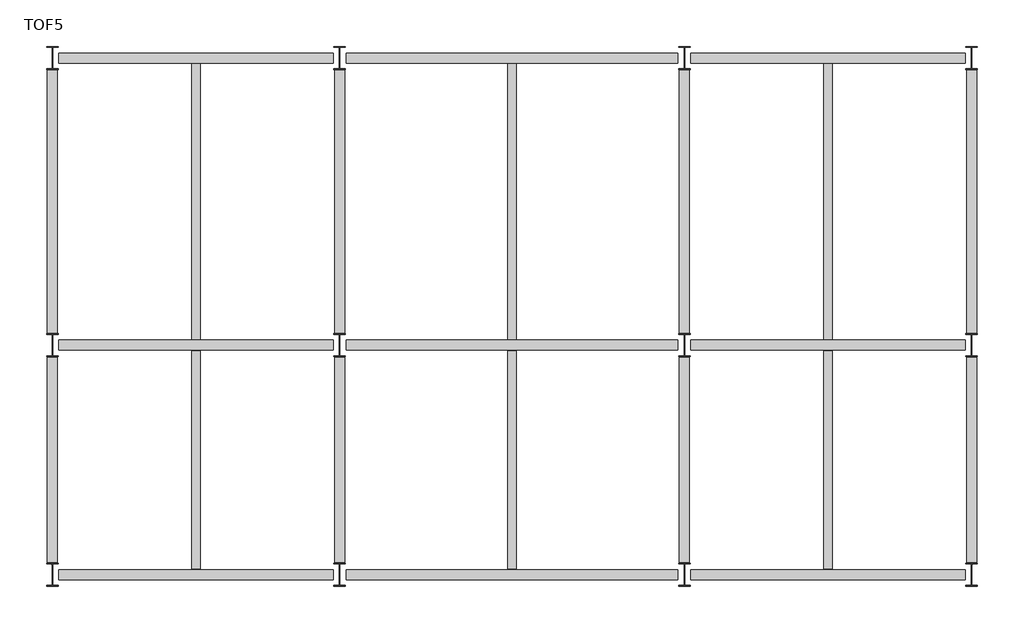
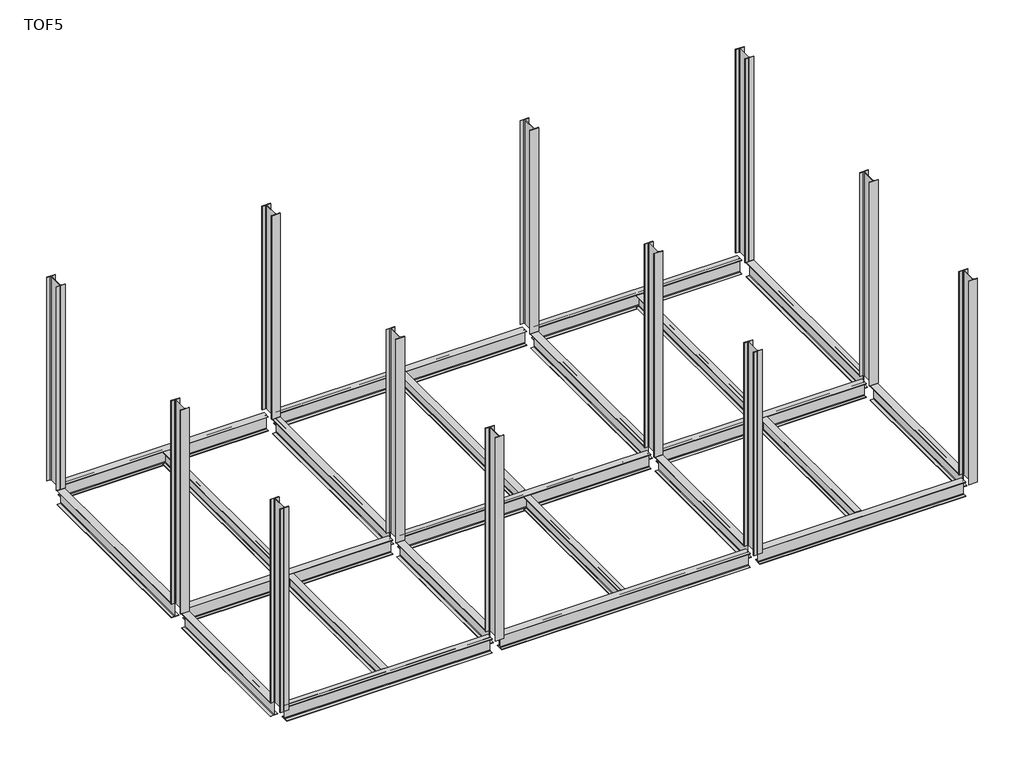
# One storey: 23 beams, 12 columns.
"""IFC4 building model written with IfcOpenShell, lengths in millimetres."""

import ifcopenshell
import ifcopenshell.guid

model = None  # the IFC model being written
_history = None  # IfcOwnerHistory: only IFC2X3 demands one
_inside = {}  # id of a spatial element -> (the spatial element, [elements in it])
_under = {}  # id of a project, library or spatial element -> (it, [spatial elements below it])
_declared = {}  # id of a project -> (the project, [libraries it declares])
_typed = {}  # id of a type object -> (the type object, [elements of that type])
_made_of = {}  # id of a material, layer set ... -> (it, [elements and type objects made of it])


def new_model(schema):
    """Start an empty IFC model of exactly this schema.

    Asked for "IFC4X3", IfcOpenShell would pick the latest addendum, in which some entities
    have other attributes; the version numbers below select the first issue.
    IFC2X3 requires an IfcOwnerHistory on every rooted entity: one is made here for all.
    """
    global model, _history
    if schema == "IFC4X3":
        model = ifcopenshell.file(schema_version=(4, 3, 0, 0))
    else:
        model = ifcopenshell.file(schema=schema)
    _inside.clear()
    _under.clear()
    _declared.clear()
    _typed.clear()
    _made_of.clear()
    _history = None
    if model.schema == "IFC2X3":
        org = make("IfcOrganization", Name="unknown")
        user = make(
            "IfcPersonAndOrganization",
            ThePerson=make("IfcPerson", FamilyName="unknown"),
            TheOrganization=org,
        )
        app = make(
            "IfcApplication",
            ApplicationDeveloper=org,
            Version="unknown",
            ApplicationFullName="unknown",
            ApplicationIdentifier="unknown",
        )
        _history = make(
            "IfcOwnerHistory",
            OwningUser=user,
            OwningApplication=app,
            ChangeAction="ADDED",
            CreationDate=0,
        )
    return model


def make(cls, **values):
    """One entity of the class cls with the attributes given. An attribute that is None is left unset."""
    return model.create_entity(
        cls, **{name: value for name, value in values.items() if value is not None}
    )


def rooted(cls, **values):
    """An entity with a GlobalId (a new one), such as an element, a storey or a relation."""
    return make(cls, GlobalId=ifcopenshell.guid.new(), OwnerHistory=_history, **values)


def si_unit(unit_type, name, prefix=None):
    """IfcSIUnit, for example si_unit("LENGTHUNIT", "METRE", prefix="MILLI")."""
    return make("IfcSIUnit", UnitType=unit_type, Prefix=prefix, Name=name)


def assignment(units):
    """IfcUnitAssignment: the units of a project."""
    return None if units is None else make("IfcUnitAssignment", Units=units)


def point(xyz):
    """IfcCartesianPoint."""
    return None if xyz is None else make("IfcCartesianPoint", Coordinates=xyz)


def direction(xyz):
    """IfcDirection."""
    return None if xyz is None else make("IfcDirection", DirectionRatios=xyz)


def frame(location, z_axis=None, x_axis=None):
    """IfcAxis2Placement3D, a coordinate frame: its origin and axes. An axis left out is left unset."""
    return make(
        "IfcAxis2Placement3D",
        Location=point(location),
        Axis=direction(z_axis),
        RefDirection=direction(x_axis),
    )


def frame_2d(location, x_axis=None):
    """IfcAxis2Placement2D, a coordinate frame in the plane: its origin and x axis."""
    return make(
        "IfcAxis2Placement2D", Location=point(location), RefDirection=direction(x_axis)
    )


def origin():
    """The frame at (0, 0, 0) with its axes left unset."""
    return frame((0.0, 0.0, 0.0))


def place(relative_to, where):
    """IfcLocalPlacement: puts the frame where relative to a parent placement (None: the world)."""
    return make(
        "IfcLocalPlacement", PlacementRelTo=relative_to, RelativePlacement=where
    )


def context(
    kind, dimensions, precision=None, world=None, true_north=None, identifier=None
):
    """IfcGeometricRepresentationContext, for example the 3D "Model" context."""
    return make(
        "IfcGeometricRepresentationContext",
        ContextIdentifier=identifier,
        ContextType=kind,
        CoordinateSpaceDimension=dimensions,
        Precision=precision,
        WorldCoordinateSystem=world,
        TrueNorth=true_north,
    )


def project(units=None, contexts=None):
    """IfcProject with its units and contexts."""
    return rooted(
        "IfcProject",
        Name="project",
        RepresentationContexts=contexts,
        UnitsInContext=assignment(units),
    )


def spatial(cls, under=None, at=None, **own):
    """A site, building, storey or space (cls), placed at a placement, below another one or the project."""
    s = rooted(cls, ObjectPlacement=at, **own)
    if under is not None:
        _under.setdefault(under.id(), (under, []))[1].append(s)
    return s


def polyline(points):
    """IfcPolyline through the points."""
    return make("IfcPolyline", Points=[point(p) for p in points])


def circle_curve(where, radius):
    """IfcCircle in the frame where."""
    return make("IfcCircle", Position=where, Radius=radius)


def trimmed(basis, trim1, trim2, sense, master):
    """IfcTrimmedCurve: the piece of a basis curve between two trims."""
    return make(
        "IfcTrimmedCurve",
        BasisCurve=basis,
        Trim1=trim1,
        Trim2=trim2,
        SenseAgreement=sense,
        MasterRepresentation=master,
    )


def segment(curve, same_sense, transition):
    """IfcCompositeCurveSegment."""
    return make(
        "IfcCompositeCurveSegment",
        Transition=transition,
        SameSense=same_sense,
        ParentCurve=curve,
    )


def composite_curve(segments, self_intersect=None):
    """IfcCompositeCurve: segments joined end to end."""
    return make("IfcCompositeCurve", Segments=segments, SelfIntersect=self_intersect)


def outline(outer, holes=None, kind="AREA"):
    """IfcArbitraryClosedProfileDef: a profile drawn as a closed curve; with holes, ...WithVoids."""
    if holes is None:
        return make("IfcArbitraryClosedProfileDef", ProfileType=kind, OuterCurve=outer)
    return make(
        "IfcArbitraryProfileDefWithVoids",
        ProfileType=kind,
        OuterCurve=outer,
        InnerCurves=holes,
    )


def extrude(swept, where, along, depth):
    """IfcExtrudedAreaSolid: the profile swept, set in the frame where, extruded along a direction by depth."""
    return make(
        "IfcExtrudedAreaSolid",
        SweptArea=swept,
        Position=where,
        ExtrudedDirection=direction(along),
        Depth=depth,
    )


def shape(context_of_items, identifier, shape_type, items):
    """IfcShapeRepresentation: the items that make up one representation, for example the "Body"."""
    return make(
        "IfcShapeRepresentation",
        ContextOfItems=context_of_items,
        RepresentationIdentifier=identifier,
        RepresentationType=shape_type,
        Items=items,
    )


def source(mapping_origin, context_of_items, identifier, shape_type, items):
    """IfcRepresentationMap: a shape defined once, which mapped items show again and again."""
    return make(
        "IfcRepresentationMap",
        MappingOrigin=mapping_origin,
        MappedRepresentation=shape(context_of_items, identifier, shape_type, items),
    )


def transform(
    local_origin,
    x_axis=None,
    y_axis=None,
    z_axis=None,
    scale=None,
    scale2=None,
    scale3=None,
    uniform=True,
):
    """IfcCartesianTransformationOperator3D, or its non-uniform kind. x_axis, y_axis, z_axis: its Axis1, 2, 3."""
    if uniform:
        return make(
            "IfcCartesianTransformationOperator3D",
            Axis1=direction(x_axis),
            Axis2=direction(y_axis),
            LocalOrigin=point(local_origin),
            Scale=scale,
            Axis3=direction(z_axis),
        )
    return make(
        "IfcCartesianTransformationOperator3DnonUniform",
        Axis1=direction(x_axis),
        Axis2=direction(y_axis),
        LocalOrigin=point(local_origin),
        Scale=scale,
        Axis3=direction(z_axis),
        Scale2=scale2,
        Scale3=scale3,
    )


def mapped(mapping_source, mapping_target):
    """IfcMappedItem: shows the shape of a source again, moved by a transform."""
    return make(
        "IfcMappedItem", MappingSource=mapping_source, MappingTarget=mapping_target
    )


def made_of(thing, what):
    """Note that an element or type object is made of a material, layer set ...; save() writes the relation."""
    if what is not None:
        _made_of.setdefault(what.id(), (what, []))[1].append(thing)
    return thing


def element(
    cls,
    number,
    at=None,
    inside=None,
    cuts=None,
    type_object=None,
    material=None,
    context=None,
    identifier="Body",
    shape_type=None,
    held_by="IfcProductDefinitionShape",
    body=None,
    shapes=None,
    **own,
):
    """One element of the class cls, such as IfcWall. Its Tag is "e" and its number.

    at: its placement. inside: the storey or other place that contains it. cuts: it is an
    opening in that element (IfcRelVoidsElement). A single representation is given by context,
    identifier, shape_type and body (its items); several are given by shapes. held_by: the class
    of the entity that holds the representations. save() writes the other relations.
    """
    e = rooted(cls, Tag="e%d" % number, ObjectPlacement=at, **own)
    if body is not None:
        shapes = [shape(context, identifier, shape_type, body)]
    if shapes is not None:
        e.Representation = make(held_by, Representations=shapes)
    if inside is not None:
        _inside.setdefault(inside.id(), (inside, []))[1].append(e)
    if cuts is not None:
        rooted(
            "IfcRelVoidsElement", RelatingBuildingElement=cuts, RelatedOpeningElement=e
        )
    if type_object is not None:
        _typed.setdefault(type_object.id(), (type_object, []))[1].append(e)
    return made_of(e, material)


def aggregate(whole, parts):
    """IfcRelAggregates: a whole, such as a stair, and the parts it consists of."""
    return rooted("IfcRelAggregates", RelatingObject=whole, RelatedObjects=parts)


def save(model, path):
    """Write the relations noted so far, then the file.

    IfcRelAggregates (storeys below a building ...), IfcRelContainedInSpatialStructure (elements
    in a storey), IfcRelDefinesByType, IfcRelAssociatesMaterial and IfcRelDeclares: one each for
    every whole, place, type object, material and project.
    """
    for whole, parts in _under.values():
        aggregate(whole, parts)
    for where, things in _inside.values():
        rooted(
            "IfcRelContainedInSpatialStructure",
            RelatedElements=things,
            RelatingStructure=where,
        )
    for kind, things in _typed.values():
        rooted("IfcRelDefinesByType", RelatedObjects=things, RelatingType=kind)
    for what, things in _made_of.values():
        rooted("IfcRelAssociatesMaterial", RelatedObjects=things, RelatingMaterial=what)
    for by, libraries in _declared.values():
        rooted("IfcRelDeclares", RelatingContext=by, RelatedDefinitions=libraries)
    model.write(path)


def beam_edbab3fa(model_context):
    return source(origin(), model_context, "Body", "SweptSolid", [
        extrude(outline(composite_curve([segment(polyline([(75.0, -141.0), (75.0, -150.0), (-75.0, -150.0), (-75.0, -141.0), (-16.25, -141.0)]), True, "CONTINUOUS"), segment(trimmed(circle_curve(frame_2d((-16.25, -128.0)), 13.0), [point((-16.25, -141.0))], [point((-3.25, -128.0))], True, "CARTESIAN"), True, "CONTINUOUS"), segment(polyline([(-3.25, -128.0), (-3.25, 128.0)]), True, "CONTINUOUS"), segment(trimmed(circle_curve(frame_2d((-16.25, 128.0)), 13.0), [point((-3.25, 128.0))], [point((-16.25, 141.0))], True, "CARTESIAN"), True, "CONTINUOUS"), segment(polyline([(-16.25, 141.0), (-75.0, 141.0), (-75.0, 150.0), (75.0, 150.0), (75.0, 141.0), (16.25, 141.0)]), True, "CONTINUOUS"), segment(trimmed(circle_curve(frame_2d((16.25, 128.0)), 13.0), [point((16.25, 141.0))], [point((3.25, 128.0))], True, "CARTESIAN"), True, "CONTINUOUS"), segment(polyline([(3.25, 128.0), (3.25, -128.0)]), True, "CONTINUOUS"), segment(trimmed(circle_curve(frame_2d((16.25, -128.0)), 13.0), [point((3.25, -128.0))], [point((16.25, -141.0))], True, "CARTESIAN"), True, "CONTINUOUS"), segment(polyline([(16.25, -141.0), (75.0, -141.0)]), True, "CONTINUOUS")], self_intersect=False)), frame((-1899.8, 0.0, 0.0), z_axis=(1.0, 0.0, 0.0), x_axis=(0.0, 1.0, 0.0)), (0.0, 0.0, 1.0), 3799.6),
    ])


def beam_c00964ff(model_context):
    return source(origin(), model_context, "Body", "SweptSolid", [
        extrude(outline(composite_curve([segment(polyline([(75.0, -141.0), (75.0, -150.0), (-75.0, -150.0), (-75.0, -141.0), (-16.25, -141.0)]), True, "CONTINUOUS"), segment(trimmed(circle_curve(frame_2d((-16.25, -128.0)), 13.0), [point((-16.25, -141.0))], [point((-3.25, -128.0))], True, "CARTESIAN"), True, "CONTINUOUS"), segment(polyline([(-3.25, -128.0), (-3.25, 128.0)]), True, "CONTINUOUS"), segment(trimmed(circle_curve(frame_2d((-16.25, 128.0)), 13.0), [point((-3.25, 128.0))], [point((-16.25, 141.0))], True, "CARTESIAN"), True, "CONTINUOUS"), segment(polyline([(-16.25, 141.0), (-75.0, 141.0), (-75.0, 150.0), (75.0, 150.0), (75.0, 141.0), (16.25, 141.0)]), True, "CONTINUOUS"), segment(trimmed(circle_curve(frame_2d((16.25, 128.0)), 13.0), [point((16.25, 141.0))], [point((3.25, 128.0))], True, "CARTESIAN"), True, "CONTINUOUS"), segment(polyline([(3.25, 128.0), (3.25, -128.0)]), True, "CONTINUOUS"), segment(trimmed(circle_curve(frame_2d((16.25, -128.0)), 13.0), [point((3.25, -128.0))], [point((16.25, -141.0))], True, "CARTESIAN"), True, "CONTINUOUS"), segment(polyline([(16.25, -141.0), (75.0, -141.0)]), True, "CONTINUOUS")], self_intersect=False)), frame((-2399.8, 0.0, 0.0), z_axis=(1.0, 0.0, 0.0), x_axis=(0.0, 1.0, 0.0)), (0.0, 0.0, 1.0), 4799.6),
    ])


def beam_74d50635(model_context):
    return source(origin(), model_context, "Body", "SweptSolid", [
        extrude(outline(composite_curve([segment(polyline([(87.5, -164.0), (87.5, -175.0), (-87.5, -175.0), (-87.5, -164.0), (-17.5, -164.0)]), True, "CONTINUOUS"), segment(trimmed(circle_curve(frame_2d((-17.5, -150.0)), 14.0), [point((-17.5, -164.0))], [point((-3.5, -150.0))], True, "CARTESIAN"), True, "CONTINUOUS"), segment(polyline([(-3.5, -150.0), (-3.5, 150.0)]), True, "CONTINUOUS"), segment(trimmed(circle_curve(frame_2d((-17.5, 150.0)), 14.0), [point((-3.5, 150.0))], [point((-17.5, 164.0))], True, "CARTESIAN"), True, "CONTINUOUS"), segment(polyline([(-17.5, 164.0), (-87.5, 164.0), (-87.5, 175.0), (87.5, 175.0), (87.5, 164.0), (17.5, 164.0)]), True, "CONTINUOUS"), segment(trimmed(circle_curve(frame_2d((17.5, 150.0)), 14.0), [point((17.5, 164.0))], [point((3.5, 150.0))], True, "CARTESIAN"), True, "CONTINUOUS"), segment(polyline([(3.5, 150.0), (3.5, -150.0)]), True, "CONTINUOUS"), segment(trimmed(circle_curve(frame_2d((17.5, -150.0)), 14.0), [point((3.5, -150.0))], [point((17.5, -164.0))], True, "CARTESIAN"), True, "CONTINUOUS"), segment(polyline([(17.5, -164.0), (87.5, -164.0)]), True, "CONTINUOUS")], self_intersect=False)), frame((-2387.3, 0.0, 0.0), z_axis=(1.0, 0.0, 0.0), x_axis=(0.0, 1.0, 0.0)), (0.0, 0.0, 1.0), 4774.6),
    ])


def beam_3a5a8fac(model_context):
    return source(origin(), model_context, "Body", "SweptSolid", [
        extrude(outline(composite_curve([segment(polyline([(87.5, -164.0), (87.5, -175.0), (-87.5, -175.0), (-87.5, -164.0), (-17.5, -164.0)]), True, "CONTINUOUS"), segment(trimmed(circle_curve(frame_2d((-17.5, -150.0)), 14.0), [point((-17.5, -164.0))], [point((-3.5, -150.0))], True, "CARTESIAN"), True, "CONTINUOUS"), segment(polyline([(-3.5, -150.0), (-3.5, 150.0)]), True, "CONTINUOUS"), segment(trimmed(circle_curve(frame_2d((-17.5, 150.0)), 14.0), [point((-3.5, 150.0))], [point((-17.5, 164.0))], True, "CARTESIAN"), True, "CONTINUOUS"), segment(polyline([(-17.5, 164.0), (-87.5, 164.0), (-87.5, 175.0), (87.5, 175.0), (87.5, 164.0), (17.5, 164.0)]), True, "CONTINUOUS"), segment(trimmed(circle_curve(frame_2d((17.5, 150.0)), 14.0), [point((17.5, 164.0))], [point((3.5, 150.0))], True, "CARTESIAN"), True, "CONTINUOUS"), segment(polyline([(3.5, 150.0), (3.5, -150.0)]), True, "CONTINUOUS"), segment(trimmed(circle_curve(frame_2d((17.5, -150.0)), 14.0), [point((3.5, -150.0))], [point((17.5, -164.0))], True, "CARTESIAN"), True, "CONTINUOUS"), segment(polyline([(17.5, -164.0), (87.5, -164.0)]), True, "CONTINUOUS")], self_intersect=False)), frame((-2887.3, 0.0, 0.0), z_axis=(1.0, 0.0, 0.0), x_axis=(0.0, 1.0, 0.0)), (0.0, 0.0, 1.0), 5774.6),
    ])


def beam_edcef29c(model_context):
    return source(origin(), model_context, "Body", "SweptSolid", [
        extrude(outline(composite_curve([segment(polyline([(87.5, -164.0), (87.5, -175.0), (-87.5, -175.0), (-87.5, -164.0), (-17.5, -164.0)]), True, "CONTINUOUS"), segment(trimmed(circle_curve(frame_2d((-17.5, -150.0)), 14.0), [point((-17.5, -164.0))], [point((-3.5, -150.0))], True, "CARTESIAN"), True, "CONTINUOUS"), segment(polyline([(-3.5, -150.0), (-3.5, 150.0)]), True, "CONTINUOUS"), segment(trimmed(circle_curve(frame_2d((-17.5, 150.0)), 14.0), [point((-3.5, 150.0))], [point((-17.5, 164.0))], True, "CARTESIAN"), True, "CONTINUOUS"), segment(polyline([(-17.5, 164.0), (-87.5, 164.0), (-87.5, 175.0), (87.5, 175.0), (87.5, 164.0), (17.5, 164.0)]), True, "CONTINUOUS"), segment(trimmed(circle_curve(frame_2d((17.5, 150.0)), 14.0), [point((17.5, 164.0))], [point((3.5, 150.0))], True, "CARTESIAN"), True, "CONTINUOUS"), segment(polyline([(3.5, 150.0), (3.5, -150.0)]), True, "CONTINUOUS"), segment(trimmed(circle_curve(frame_2d((17.5, -150.0)), 14.0), [point((3.5, -150.0))], [point((17.5, -164.0))], True, "CARTESIAN"), True, "CONTINUOUS"), segment(polyline([(17.5, -164.0), (87.5, -164.0)]), True, "CONTINUOUS")], self_intersect=False)), frame((-1787.3, 0.0, 0.0), z_axis=(1.0, 0.0, 0.0), x_axis=(0.0, 1.0, 0.0)), (0.0, 0.0, 1.0), 3574.6),
    ])


def beam_68894c75(model_context):
    return source(origin(), model_context, "Body", "SweptSolid", [
        extrude(outline(composite_curve([segment(polyline([(87.5, -164.0), (87.5, -175.0), (-87.5, -175.0), (-87.5, -164.0), (-17.5, -164.0)]), True, "CONTINUOUS"), segment(trimmed(circle_curve(frame_2d((-17.5, -150.0)), 14.0), [point((-17.5, -164.0))], [point((-3.5, -150.0))], True, "CARTESIAN"), True, "CONTINUOUS"), segment(polyline([(-3.5, -150.0), (-3.5, 150.0)]), True, "CONTINUOUS"), segment(trimmed(circle_curve(frame_2d((-17.5, 150.0)), 14.0), [point((-3.5, 150.0))], [point((-17.5, 164.0))], True, "CARTESIAN"), True, "CONTINUOUS"), segment(polyline([(-17.5, 164.0), (-87.5, 164.0), (-87.5, 175.0), (87.5, 175.0), (87.5, 164.0), (17.5, 164.0)]), True, "CONTINUOUS"), segment(trimmed(circle_curve(frame_2d((17.5, 150.0)), 14.0), [point((17.5, 164.0))], [point((3.5, 150.0))], True, "CARTESIAN"), True, "CONTINUOUS"), segment(polyline([(3.5, 150.0), (3.5, -150.0)]), True, "CONTINUOUS"), segment(trimmed(circle_curve(frame_2d((17.5, -150.0)), 14.0), [point((3.5, -150.0))], [point((17.5, -164.0))], True, "CARTESIAN"), True, "CONTINUOUS"), segment(polyline([(17.5, -164.0), (87.5, -164.0)]), True, "CONTINUOUS")], self_intersect=False)), frame((-2287.3, 0.0, 0.0), z_axis=(1.0, 0.0, 0.0), x_axis=(0.0, 1.0, 0.0)), (0.0, 0.0, 1.0), 4574.6),
    ])


model = new_model("IFC4")

# Units and contexts
model_context = context("Model", 3, world=origin())
ifc_project = project(units=[si_unit("LENGTHUNIT", "METRE", prefix="MILLI")], contexts=[model_context])

# Site, building, storey
site = spatial("IfcSite", under=ifc_project)
building = spatial("IfcBuilding", under=site)
storey = spatial("IfcBuildingStorey", under=building, Name="TOF5", Elevation=4000.0)

# Beams
placement = place(None, origin())
beam_shape = beam_edbab3fa(model_context)
element("IfcBeam", 1, ObjectType="0912_Steel Framing_H-KSD3502 : H_SB_AR_S02_H-300x150x6.5x9_Stair", at=placement, inside=storey, context=model_context, shape_type="MappedRepresentation", body=[
    mapped(beam_shape, transform((2500.0, 2000.0, 3850.0), x_axis=(0.0, 1.0, 0.0), y_axis=(-1.0, 0.0, 0.0), z_axis=(0.0, 0.0, 1.0))),
])
element("IfcBeam", 2, ObjectType="0912_Steel Framing_H-KSD3502 : H_SB_AR_S02_H-300x150x6.5x9_Stair", at=placement, inside=storey, context=model_context, shape_type="MappedRepresentation", body=[
    mapped(beam_shape, transform((8000.0, 2000.0, 3850.0), x_axis=(0.0, 1.0, 0.0), y_axis=(-1.0, 0.0, 0.0), z_axis=(0.0, 0.0, 1.0))),
])
element("IfcBeam", 3, ObjectType="0912_Steel Framing_H-KSD3502 : H_SB_AR_S02_H-300x150x6.5x9_Stair", at=placement, inside=storey, context=model_context, shape_type="MappedRepresentation", body=[
    mapped(beam_shape, transform((13500.0, 2000.0, 3850.0), x_axis=(0.0, 1.0, 0.0), y_axis=(-1.0, 0.0, 0.0), z_axis=(0.0, 0.0, 1.0))),
])
beam_2_shape = beam_c00964ff(model_context)
element("IfcBeam", 4, ObjectType="0912_Steel Framing_H-KSD3502 : H_SB_AR_S02_H-300x150x6.5x9_Stair", at=placement, inside=storey, context=model_context, shape_type="MappedRepresentation", body=[
    mapped(beam_2_shape, transform((2500.0, 6500.0, 3850.0), x_axis=(0.0, 1.0, 0.0), y_axis=(-1.0, 0.0, 0.0), z_axis=(0.0, 0.0, 1.0))),
])
element("IfcBeam", 5, ObjectType="0912_Steel Framing_H-KSD3502 : H_SB_AR_S02_H-300x150x6.5x9_Stair", at=placement, inside=storey, context=model_context, shape_type="MappedRepresentation", body=[
    mapped(beam_2_shape, transform((8000.0, 6500.0, 3850.0), x_axis=(0.0, 1.0, 0.0), y_axis=(-1.0, 0.0, 0.0), z_axis=(0.0, 0.0, 1.0))),
])
element("IfcBeam", 6, ObjectType="0912_Steel Framing_H-KSD3502 : H_SB_AR_S02_H-300x150x6.5x9_Stair", at=placement, inside=storey, context=model_context, shape_type="MappedRepresentation", body=[
    mapped(beam_2_shape, transform((13500.0, 6500.0, 3850.0), x_axis=(0.0, 1.0, 0.0), y_axis=(-1.0, 0.0, 0.0), z_axis=(0.0, 0.0, 1.0))),
])
beam_3_shape = beam_74d50635(model_context)
element("IfcBeam", 7, ObjectType="0912_Steel Framing_H-KSD3502 : H_SB_AR_S02_H-350x175x7x11_Platform", at=placement, inside=storey, context=model_context, shape_type="MappedRepresentation", body=[
    mapped(beam_3_shape, transform((2500.0, 0.0, 3825.0), x_axis=(1.0, 0.0, 0.0), y_axis=(0.0, 1.0, 0.0), z_axis=(0.0, 0.0, 1.0))),
])
element("IfcBeam", 8, ObjectType="0912_Steel Framing_H-KSD3502 : H_SB_AR_S02_H-350x175x7x11_Platform", at=placement, inside=storey, context=model_context, shape_type="MappedRepresentation", body=[
    mapped(beam_3_shape, transform((13500.0, 0.0, 3825.0), x_axis=(1.0, 0.0, 0.0), y_axis=(0.0, 1.0, 0.0), z_axis=(0.0, 0.0, 1.0))),
])
element("IfcBeam", 9, ObjectType="0912_Steel Framing_H-KSD3502 : H_SB_AR_S02_H-350x175x7x11_Platform", at=placement, inside=storey, context=model_context, shape_type="MappedRepresentation", body=[
    mapped(beam_3_shape, transform((2500.0, 4000.0, 3825.0), x_axis=(1.0, 0.0, 0.0), y_axis=(0.0, 1.0, 0.0), z_axis=(0.0, 0.0, 1.0))),
])
element("IfcBeam", 10, ObjectType="0912_Steel Framing_H-KSD3502 : H_SB_AR_S02_H-350x175x7x11_Platform", at=placement, inside=storey, context=model_context, shape_type="MappedRepresentation", body=[
    mapped(beam_3_shape, transform((13500.0, 4000.0, 3825.0), x_axis=(1.0, 0.0, 0.0), y_axis=(0.0, 1.0, 0.0), z_axis=(0.0, 0.0, 1.0))),
])
element("IfcBeam", 11, ObjectType="0912_Steel Framing_H-KSD3502 : H_SB_AR_S02_H-350x175x7x11_Platform", at=placement, inside=storey, context=model_context, shape_type="MappedRepresentation", body=[
    mapped(beam_3_shape, transform((2500.0, 9000.0, 3825.0), x_axis=(1.0, 0.0, 0.0), y_axis=(0.0, 1.0, 0.0), z_axis=(0.0, 0.0, 1.0))),
])
element("IfcBeam", 12, ObjectType="0912_Steel Framing_H-KSD3502 : H_SB_AR_S02_H-350x175x7x11_Platform", at=placement, inside=storey, context=model_context, shape_type="MappedRepresentation", body=[
    mapped(beam_3_shape, transform((13500.0, 9000.0, 3825.0), x_axis=(1.0, 0.0, 0.0), y_axis=(0.0, 1.0, 0.0), z_axis=(0.0, 0.0, 1.0))),
])
beam_4_shape = beam_3a5a8fac(model_context)
element("IfcBeam", 13, ObjectType="0912_Steel Framing_H-KSD3502 : H_SB_AR_S02_H-350x175x7x11_Platform", at=placement, inside=storey, context=model_context, shape_type="MappedRepresentation", body=[
    mapped(beam_4_shape, transform((8000.0, 0.0, 3825.0), x_axis=(1.0, 0.0, 0.0), y_axis=(0.0, 1.0, 0.0), z_axis=(0.0, 0.0, 1.0))),
])
element("IfcBeam", 14, ObjectType="0912_Steel Framing_H-KSD3502 : H_SB_AR_S02_H-350x175x7x11_Platform", at=placement, inside=storey, context=model_context, shape_type="MappedRepresentation", body=[
    mapped(beam_4_shape, transform((8000.0, 4000.0, 3825.0), x_axis=(1.0, 0.0, 0.0), y_axis=(0.0, 1.0, 0.0), z_axis=(0.0, 0.0, 1.0))),
])
element("IfcBeam", 15, ObjectType="0912_Steel Framing_H-KSD3502 : H_SB_AR_S02_H-350x175x7x11_Platform", at=placement, inside=storey, context=model_context, shape_type="MappedRepresentation", body=[
    mapped(beam_4_shape, transform((8000.0, 9000.0, 3825.0), x_axis=(1.0, 0.0, 0.0), y_axis=(0.0, 1.0, 0.0), z_axis=(0.0, 0.0, 1.0))),
])
beam_5_shape = beam_edcef29c(model_context)
element("IfcBeam", 16, ObjectType="0912_Steel Framing_H-KSD3502 : H_SB_AR_S02_H-350x175x7x11_Platform", at=placement, inside=storey, context=model_context, shape_type="MappedRepresentation", body=[
    mapped(beam_5_shape, transform((0.0, 2000.0, 3825.0), x_axis=(0.0, 1.0, 0.0), y_axis=(-1.0, 0.0, 0.0), z_axis=(0.0, 0.0, 1.0))),
])
element("IfcBeam", 17, ObjectType="0912_Steel Framing_H-KSD3502 : H_SB_AR_S02_H-350x175x7x11_Platform", at=placement, inside=storey, context=model_context, shape_type="MappedRepresentation", body=[
    mapped(beam_5_shape, transform((5000.0, 2000.0, 3825.0), x_axis=(0.0, 1.0, 0.0), y_axis=(-1.0, 0.0, 0.0), z_axis=(0.0, 0.0, 1.0))),
])
element("IfcBeam", 18, ObjectType="0912_Steel Framing_H-KSD3502 : H_SB_AR_S02_H-350x175x7x11_Platform", at=placement, inside=storey, context=model_context, shape_type="MappedRepresentation", body=[
    mapped(beam_5_shape, transform((11000.0, 2000.0, 3825.0), x_axis=(0.0, 1.0, 0.0), y_axis=(-1.0, 0.0, 0.0), z_axis=(0.0, 0.0, 1.0))),
])
element("IfcBeam", 19, ObjectType="0912_Steel Framing_H-KSD3502 : H_SB_AR_S02_H-350x175x7x11_Platform", at=placement, inside=storey, context=model_context, shape_type="MappedRepresentation", body=[
    mapped(beam_5_shape, transform((16000.0, 2000.0, 3825.0), x_axis=(0.0, 1.0, 0.0), y_axis=(-1.0, 0.0, 0.0), z_axis=(0.0, 0.0, 1.0))),
])
beam_6_shape = beam_68894c75(model_context)
element("IfcBeam", 20, ObjectType="0912_Steel Framing_H-KSD3502 : H_SB_AR_S02_H-350x175x7x11_Platform", at=placement, inside=storey, context=model_context, shape_type="MappedRepresentation", body=[
    mapped(beam_6_shape, transform((0.0, 6500.0, 3825.0), x_axis=(0.0, 1.0, 0.0), y_axis=(-1.0, 0.0, 0.0), z_axis=(0.0, 0.0, 1.0))),
])
element("IfcBeam", 21, ObjectType="0912_Steel Framing_H-KSD3502 : H_SB_AR_S02_H-350x175x7x11_Platform", at=placement, inside=storey, context=model_context, shape_type="MappedRepresentation", body=[
    mapped(beam_6_shape, transform((5000.0, 6500.0, 3825.0), x_axis=(0.0, 1.0, 0.0), y_axis=(-1.0, 0.0, 0.0), z_axis=(0.0, 0.0, 1.0))),
])
element("IfcBeam", 22, ObjectType="0912_Steel Framing_H-KSD3502 : H_SB_AR_S02_H-350x175x7x11_Platform", at=placement, inside=storey, context=model_context, shape_type="MappedRepresentation", body=[
    mapped(beam_6_shape, transform((11000.0, 6500.0, 3825.0), x_axis=(0.0, 1.0, 0.0), y_axis=(-1.0, 0.0, 0.0), z_axis=(0.0, 0.0, 1.0))),
])
element("IfcBeam", 23, ObjectType="0912_Steel Framing_H-KSD3502 : H_SB_AR_S02_H-350x175x7x11_Platform", at=placement, inside=storey, context=model_context, shape_type="MappedRepresentation", body=[
    mapped(beam_6_shape, transform((16000.0, 6500.0, 3825.0), x_axis=(0.0, 1.0, 0.0), y_axis=(-1.0, 0.0, 0.0), z_axis=(0.0, 0.0, 1.0))),
])

# Columns
element("IfcColumn", 24, ObjectType="Steel Column_H_KSD3502 : H_SC_AR_S01_H-400x200x8x13", at=placement, inside=storey, context=model_context, shape_type="SweptSolid", body=[
    extrude(outline(composite_curve([segment(polyline([(100.0, 200.0), (100.0, 187.0), (20.0, 187.0)]), True, "CONTINUOUS"), segment(trimmed(circle_curve(frame_2d((20.0, 171.0)), 16.0), [point((20.0, 187.0))], [point((4.0, 171.0))], True, "CARTESIAN"), True, "CONTINUOUS"), segment(polyline([(4.0, 171.0), (4.0, -171.0)]), True, "CONTINUOUS"), segment(trimmed(circle_curve(frame_2d((20.0, -171.0)), 16.0), [point((4.0, -171.0))], [point((20.0, -187.0))], True, "CARTESIAN"), True, "CONTINUOUS"), segment(polyline([(20.0, -187.0), (100.0, -187.0), (100.0, -200.0), (-100.0, -200.0), (-100.0, -187.0), (-20.0, -187.0)]), True, "CONTINUOUS"), segment(trimmed(circle_curve(frame_2d((-20.0, -171.0)), 16.0), [point((-20.0, -187.0))], [point((-4.0, -171.0))], True, "CARTESIAN"), True, "CONTINUOUS"), segment(polyline([(-4.0, -171.0), (-4.0, 171.0)]), True, "CONTINUOUS"), segment(trimmed(circle_curve(frame_2d((-20.0, 171.0)), 16.0), [point((-4.0, 171.0))], [point((-20.0, 187.0))], True, "CARTESIAN"), True, "CONTINUOUS"), segment(polyline([(-20.0, 187.0), (-100.0, 187.0), (-100.0, 200.0), (100.0, 200.0)]), True, "CONTINUOUS")], self_intersect=False)), frame((0.0, 0.0, 4000.0), z_axis=(0.0, 0.0, 1.0), x_axis=(1.0, 0.0, 0.0)), (0.0, 0.0, 1.0), 5000.0),
])
element("IfcColumn", 25, ObjectType="Steel Column_H_KSD3502 : H_SC_AR_S01_H-400x200x8x13", at=placement, inside=storey, context=model_context, shape_type="SweptSolid", body=[
    extrude(outline(composite_curve([segment(polyline([(5100.0, 200.0), (5100.0, 187.0), (5020.0, 187.0)]), True, "CONTINUOUS"), segment(trimmed(circle_curve(frame_2d((5020.0, 171.0)), 16.0), [point((5020.0, 187.0))], [point((5004.0, 171.0))], True, "CARTESIAN"), True, "CONTINUOUS"), segment(polyline([(5004.0, 171.0), (5004.0, -171.0)]), True, "CONTINUOUS"), segment(trimmed(circle_curve(frame_2d((5020.0, -171.0)), 16.0), [point((5004.0, -171.0))], [point((5020.0, -187.0))], True, "CARTESIAN"), True, "CONTINUOUS"), segment(polyline([(5020.0, -187.0), (5100.0, -187.0), (5100.0, -200.0), (4900.0, -200.0), (4900.0, -187.0), (4980.0, -187.0)]), True, "CONTINUOUS"), segment(trimmed(circle_curve(frame_2d((4980.0, -171.0)), 16.0), [point((4980.0, -187.0))], [point((4996.0, -171.0))], True, "CARTESIAN"), True, "CONTINUOUS"), segment(polyline([(4996.0, -171.0), (4996.0, 171.0)]), True, "CONTINUOUS"), segment(trimmed(circle_curve(frame_2d((4980.0, 171.0)), 16.0), [point((4996.0, 171.0))], [point((4980.0, 187.0))], True, "CARTESIAN"), True, "CONTINUOUS"), segment(polyline([(4980.0, 187.0), (4900.0, 187.0), (4900.0, 200.0), (5100.0, 200.0)]), True, "CONTINUOUS")], self_intersect=False)), frame((0.0, 0.0, 4000.0), z_axis=(0.0, 0.0, 1.0), x_axis=(1.0, 0.0, 0.0)), (0.0, 0.0, 1.0), 5000.0),
])
element("IfcColumn", 26, ObjectType="Steel Column_H_KSD3502 : H_SC_AR_S01_H-400x200x8x13", at=placement, inside=storey, context=model_context, shape_type="SweptSolid", body=[
    extrude(outline(composite_curve([segment(polyline([(11100.0, 200.0), (11100.0, 187.0), (11020.0, 187.0)]), True, "CONTINUOUS"), segment(trimmed(circle_curve(frame_2d((11020.0, 171.0)), 16.0), [point((11020.0, 187.0))], [point((11004.0, 171.0))], True, "CARTESIAN"), True, "CONTINUOUS"), segment(polyline([(11004.0, 171.0), (11004.0, -171.0)]), True, "CONTINUOUS"), segment(trimmed(circle_curve(frame_2d((11020.0, -171.0)), 16.0), [point((11004.0, -171.0))], [point((11020.0, -187.0))], True, "CARTESIAN"), True, "CONTINUOUS"), segment(polyline([(11020.0, -187.0), (11100.0, -187.0), (11100.0, -200.0), (10900.0, -200.0), (10900.0, -187.0), (10980.0, -187.0)]), True, "CONTINUOUS"), segment(trimmed(circle_curve(frame_2d((10980.0, -171.0)), 16.0), [point((10980.0, -187.0))], [point((10996.0, -171.0))], True, "CARTESIAN"), True, "CONTINUOUS"), segment(polyline([(10996.0, -171.0), (10996.0, 171.0)]), True, "CONTINUOUS"), segment(trimmed(circle_curve(frame_2d((10980.0, 171.0)), 16.0), [point((10996.0, 171.0))], [point((10980.0, 187.0))], True, "CARTESIAN"), True, "CONTINUOUS"), segment(polyline([(10980.0, 187.0), (10900.0, 187.0), (10900.0, 200.0), (11100.0, 200.0)]), True, "CONTINUOUS")], self_intersect=False)), frame((0.0, 0.0, 4000.0), z_axis=(0.0, 0.0, 1.0), x_axis=(1.0, 0.0, 0.0)), (0.0, 0.0, 1.0), 5000.0),
])
element("IfcColumn", 27, ObjectType="Steel Column_H_KSD3502 : H_SC_AR_S01_H-400x200x8x13", at=placement, inside=storey, context=model_context, shape_type="SweptSolid", body=[
    extrude(outline(composite_curve([segment(polyline([(16100.0, 200.0), (16100.0, 187.0), (16020.0, 187.0)]), True, "CONTINUOUS"), segment(trimmed(circle_curve(frame_2d((16020.0, 171.0)), 16.0), [point((16020.0, 187.0))], [point((16004.0, 171.0))], True, "CARTESIAN"), True, "CONTINUOUS"), segment(polyline([(16004.0, 171.0), (16004.0, -171.0)]), True, "CONTINUOUS"), segment(trimmed(circle_curve(frame_2d((16020.0, -171.0)), 16.0), [point((16004.0, -171.0))], [point((16020.0, -187.0))], True, "CARTESIAN"), True, "CONTINUOUS"), segment(polyline([(16020.0, -187.0), (16100.0, -187.0), (16100.0, -200.0), (15900.0, -200.0), (15900.0, -187.0), (15980.0, -187.0)]), True, "CONTINUOUS"), segment(trimmed(circle_curve(frame_2d((15980.0, -171.0)), 16.0), [point((15980.0, -187.0))], [point((15996.0, -171.0))], True, "CARTESIAN"), True, "CONTINUOUS"), segment(polyline([(15996.0, -171.0), (15996.0, 171.0)]), True, "CONTINUOUS"), segment(trimmed(circle_curve(frame_2d((15980.0, 171.0)), 16.0), [point((15996.0, 171.0))], [point((15980.0, 187.0))], True, "CARTESIAN"), True, "CONTINUOUS"), segment(polyline([(15980.0, 187.0), (15900.0, 187.0), (15900.0, 200.0), (16100.0, 200.0)]), True, "CONTINUOUS")], self_intersect=False)), frame((0.0, 0.0, 4000.0), z_axis=(0.0, 0.0, 1.0), x_axis=(1.0, 0.0, 0.0)), (0.0, 0.0, 1.0), 5000.0),
])
element("IfcColumn", 28, ObjectType="Steel Column_H_KSD3502 : H_SC_AR_S01_H-400x200x8x13", at=placement, inside=storey, context=model_context, shape_type="SweptSolid", body=[
    extrude(outline(composite_curve([segment(polyline([(100.0, 4200.0), (100.0, 4187.0), (20.0, 4187.0)]), True, "CONTINUOUS"), segment(trimmed(circle_curve(frame_2d((20.0, 4171.0)), 16.0), [point((20.0, 4187.0))], [point((4.0, 4171.0))], True, "CARTESIAN"), True, "CONTINUOUS"), segment(polyline([(4.0, 4171.0), (4.0, 3829.0)]), True, "CONTINUOUS"), segment(trimmed(circle_curve(frame_2d((20.0, 3829.0)), 16.0), [point((4.0, 3829.0))], [point((20.0, 3813.0))], True, "CARTESIAN"), True, "CONTINUOUS"), segment(polyline([(20.0, 3813.0), (100.0, 3813.0), (100.0, 3800.0), (-100.0, 3800.0), (-100.0, 3813.0), (-20.0, 3813.0)]), True, "CONTINUOUS"), segment(trimmed(circle_curve(frame_2d((-20.0, 3829.0)), 16.0), [point((-20.0, 3813.0))], [point((-4.0, 3829.0))], True, "CARTESIAN"), True, "CONTINUOUS"), segment(polyline([(-4.0, 3829.0), (-4.0, 4171.0)]), True, "CONTINUOUS"), segment(trimmed(circle_curve(frame_2d((-20.0, 4171.0)), 16.0), [point((-4.0, 4171.0))], [point((-20.0, 4187.0))], True, "CARTESIAN"), True, "CONTINUOUS"), segment(polyline([(-20.0, 4187.0), (-100.0, 4187.0), (-100.0, 4200.0), (100.0, 4200.0)]), True, "CONTINUOUS")], self_intersect=False)), frame((0.0, 0.0, 4000.0), z_axis=(0.0, 0.0, 1.0), x_axis=(1.0, 0.0, 0.0)), (0.0, 0.0, 1.0), 5000.0),
])
element("IfcColumn", 29, ObjectType="Steel Column_H_KSD3502 : H_SC_AR_S01_H-400x200x8x13", at=placement, inside=storey, context=model_context, shape_type="SweptSolid", body=[
    extrude(outline(composite_curve([segment(polyline([(5100.0, 4200.0), (5100.0, 4187.0), (5020.0, 4187.0)]), True, "CONTINUOUS"), segment(trimmed(circle_curve(frame_2d((5020.0, 4171.0)), 16.0), [point((5020.0, 4187.0))], [point((5004.0, 4171.0))], True, "CARTESIAN"), True, "CONTINUOUS"), segment(polyline([(5004.0, 4171.0), (5004.0, 3829.0)]), True, "CONTINUOUS"), segment(trimmed(circle_curve(frame_2d((5020.0, 3829.0)), 16.0), [point((5004.0, 3829.0))], [point((5020.0, 3813.0))], True, "CARTESIAN"), True, "CONTINUOUS"), segment(polyline([(5020.0, 3813.0), (5100.0, 3813.0), (5100.0, 3800.0), (4900.0, 3800.0), (4900.0, 3813.0), (4980.0, 3813.0)]), True, "CONTINUOUS"), segment(trimmed(circle_curve(frame_2d((4980.0, 3829.0)), 16.0), [point((4980.0, 3813.0))], [point((4996.0, 3829.0))], True, "CARTESIAN"), True, "CONTINUOUS"), segment(polyline([(4996.0, 3829.0), (4996.0, 4171.0)]), True, "CONTINUOUS"), segment(trimmed(circle_curve(frame_2d((4980.0, 4171.0)), 16.0), [point((4996.0, 4171.0))], [point((4980.0, 4187.0))], True, "CARTESIAN"), True, "CONTINUOUS"), segment(polyline([(4980.0, 4187.0), (4900.0, 4187.0), (4900.0, 4200.0), (5100.0, 4200.0)]), True, "CONTINUOUS")], self_intersect=False)), frame((0.0, 0.0, 4000.0), z_axis=(0.0, 0.0, 1.0), x_axis=(1.0, 0.0, 0.0)), (0.0, 0.0, 1.0), 5000.0),
])
element("IfcColumn", 30, ObjectType="Steel Column_H_KSD3502 : H_SC_AR_S01_H-400x200x8x13", at=placement, inside=storey, context=model_context, shape_type="SweptSolid", body=[
    extrude(outline(composite_curve([segment(polyline([(11100.0, 4200.0), (11100.0, 4187.0), (11020.0, 4187.0)]), True, "CONTINUOUS"), segment(trimmed(circle_curve(frame_2d((11020.0, 4171.0)), 16.0), [point((11020.0, 4187.0))], [point((11004.0, 4171.0))], True, "CARTESIAN"), True, "CONTINUOUS"), segment(polyline([(11004.0, 4171.0), (11004.0, 3829.0)]), True, "CONTINUOUS"), segment(trimmed(circle_curve(frame_2d((11020.0, 3829.0)), 16.0), [point((11004.0, 3829.0))], [point((11020.0, 3813.0))], True, "CARTESIAN"), True, "CONTINUOUS"), segment(polyline([(11020.0, 3813.0), (11100.0, 3813.0), (11100.0, 3800.0), (10900.0, 3800.0), (10900.0, 3813.0), (10980.0, 3813.0)]), True, "CONTINUOUS"), segment(trimmed(circle_curve(frame_2d((10980.0, 3829.0)), 16.0), [point((10980.0, 3813.0))], [point((10996.0, 3829.0))], True, "CARTESIAN"), True, "CONTINUOUS"), segment(polyline([(10996.0, 3829.0), (10996.0, 4171.0)]), True, "CONTINUOUS"), segment(trimmed(circle_curve(frame_2d((10980.0, 4171.0)), 16.0), [point((10996.0, 4171.0))], [point((10980.0, 4187.0))], True, "CARTESIAN"), True, "CONTINUOUS"), segment(polyline([(10980.0, 4187.0), (10900.0, 4187.0), (10900.0, 4200.0), (11100.0, 4200.0)]), True, "CONTINUOUS")], self_intersect=False)), frame((0.0, 0.0, 4000.0), z_axis=(0.0, 0.0, 1.0), x_axis=(1.0, 0.0, 0.0)), (0.0, 0.0, 1.0), 5000.0),
])
element("IfcColumn", 31, ObjectType="Steel Column_H_KSD3502 : H_SC_AR_S01_H-400x200x8x13", at=placement, inside=storey, context=model_context, shape_type="SweptSolid", body=[
    extrude(outline(composite_curve([segment(polyline([(16100.0, 4200.0), (16100.0, 4187.0), (16020.0, 4187.0)]), True, "CONTINUOUS"), segment(trimmed(circle_curve(frame_2d((16020.0, 4171.0)), 16.0), [point((16020.0, 4187.0))], [point((16004.0, 4171.0))], True, "CARTESIAN"), True, "CONTINUOUS"), segment(polyline([(16004.0, 4171.0), (16004.0, 3829.0)]), True, "CONTINUOUS"), segment(trimmed(circle_curve(frame_2d((16020.0, 3829.0)), 16.0), [point((16004.0, 3829.0))], [point((16020.0, 3813.0))], True, "CARTESIAN"), True, "CONTINUOUS"), segment(polyline([(16020.0, 3813.0), (16100.0, 3813.0), (16100.0, 3800.0), (15900.0, 3800.0), (15900.0, 3813.0), (15980.0, 3813.0)]), True, "CONTINUOUS"), segment(trimmed(circle_curve(frame_2d((15980.0, 3829.0)), 16.0), [point((15980.0, 3813.0))], [point((15996.0, 3829.0))], True, "CARTESIAN"), True, "CONTINUOUS"), segment(polyline([(15996.0, 3829.0), (15996.0, 4171.0)]), True, "CONTINUOUS"), segment(trimmed(circle_curve(frame_2d((15980.0, 4171.0)), 16.0), [point((15996.0, 4171.0))], [point((15980.0, 4187.0))], True, "CARTESIAN"), True, "CONTINUOUS"), segment(polyline([(15980.0, 4187.0), (15900.0, 4187.0), (15900.0, 4200.0), (16100.0, 4200.0)]), True, "CONTINUOUS")], self_intersect=False)), frame((0.0, 0.0, 4000.0), z_axis=(0.0, 0.0, 1.0), x_axis=(1.0, 0.0, 0.0)), (0.0, 0.0, 1.0), 5000.0),
])
element("IfcColumn", 32, ObjectType="Steel Column_H_KSD3502 : H_SC_AR_S01_H-400x200x8x13", at=placement, inside=storey, context=model_context, shape_type="SweptSolid", body=[
    extrude(outline(composite_curve([segment(polyline([(100.0, 9200.0), (100.0, 9187.0), (20.0, 9187.0)]), True, "CONTINUOUS"), segment(trimmed(circle_curve(frame_2d((20.0, 9171.0)), 16.0), [point((20.0, 9187.0))], [point((4.0, 9171.0))], True, "CARTESIAN"), True, "CONTINUOUS"), segment(polyline([(4.0, 9171.0), (4.0, 8829.0)]), True, "CONTINUOUS"), segment(trimmed(circle_curve(frame_2d((20.0, 8829.0)), 16.0), [point((4.0, 8829.0))], [point((20.0, 8813.0))], True, "CARTESIAN"), True, "CONTINUOUS"), segment(polyline([(20.0, 8813.0), (100.0, 8813.0), (100.0, 8800.0), (-100.0, 8800.0), (-100.0, 8813.0), (-20.0, 8813.0)]), True, "CONTINUOUS"), segment(trimmed(circle_curve(frame_2d((-20.0, 8829.0)), 16.0), [point((-20.0, 8813.0))], [point((-4.0, 8829.0))], True, "CARTESIAN"), True, "CONTINUOUS"), segment(polyline([(-4.0, 8829.0), (-4.0, 9171.0)]), True, "CONTINUOUS"), segment(trimmed(circle_curve(frame_2d((-20.0, 9171.0)), 16.0), [point((-4.0, 9171.0))], [point((-20.0, 9187.0))], True, "CARTESIAN"), True, "CONTINUOUS"), segment(polyline([(-20.0, 9187.0), (-100.0, 9187.0), (-100.0, 9200.0), (100.0, 9200.0)]), True, "CONTINUOUS")], self_intersect=False)), frame((0.0, 0.0, 4000.0), z_axis=(0.0, 0.0, 1.0), x_axis=(1.0, 0.0, 0.0)), (0.0, 0.0, 1.0), 5000.0),
])
element("IfcColumn", 33, ObjectType="Steel Column_H_KSD3502 : H_SC_AR_S01_H-400x200x8x13", at=placement, inside=storey, context=model_context, shape_type="SweptSolid", body=[
    extrude(outline(composite_curve([segment(polyline([(5100.0, 9200.0), (5100.0, 9187.0), (5020.0, 9187.0)]), True, "CONTINUOUS"), segment(trimmed(circle_curve(frame_2d((5020.0, 9171.0)), 16.0), [point((5020.0, 9187.0))], [point((5004.0, 9171.0))], True, "CARTESIAN"), True, "CONTINUOUS"), segment(polyline([(5004.0, 9171.0), (5004.0, 8829.0)]), True, "CONTINUOUS"), segment(trimmed(circle_curve(frame_2d((5020.0, 8829.0)), 16.0), [point((5004.0, 8829.0))], [point((5020.0, 8813.0))], True, "CARTESIAN"), True, "CONTINUOUS"), segment(polyline([(5020.0, 8813.0), (5100.0, 8813.0), (5100.0, 8800.0), (4900.0, 8800.0), (4900.0, 8813.0), (4980.0, 8813.0)]), True, "CONTINUOUS"), segment(trimmed(circle_curve(frame_2d((4980.0, 8829.0)), 16.0), [point((4980.0, 8813.0))], [point((4996.0, 8829.0))], True, "CARTESIAN"), True, "CONTINUOUS"), segment(polyline([(4996.0, 8829.0), (4996.0, 9171.0)]), True, "CONTINUOUS"), segment(trimmed(circle_curve(frame_2d((4980.0, 9171.0)), 16.0), [point((4996.0, 9171.0))], [point((4980.0, 9187.0))], True, "CARTESIAN"), True, "CONTINUOUS"), segment(polyline([(4980.0, 9187.0), (4900.0, 9187.0), (4900.0, 9200.0), (5100.0, 9200.0)]), True, "CONTINUOUS")], self_intersect=False)), frame((0.0, 0.0, 4000.0), z_axis=(0.0, 0.0, 1.0), x_axis=(1.0, 0.0, 0.0)), (0.0, 0.0, 1.0), 5000.0),
])
element("IfcColumn", 34, ObjectType="Steel Column_H_KSD3502 : H_SC_AR_S01_H-400x200x8x13", at=placement, inside=storey, context=model_context, shape_type="SweptSolid", body=[
    extrude(outline(composite_curve([segment(polyline([(11100.0, 9200.0), (11100.0, 9187.0), (11020.0, 9187.0)]), True, "CONTINUOUS"), segment(trimmed(circle_curve(frame_2d((11020.0, 9171.0)), 16.0), [point((11020.0, 9187.0))], [point((11004.0, 9171.0))], True, "CARTESIAN"), True, "CONTINUOUS"), segment(polyline([(11004.0, 9171.0), (11004.0, 8829.0)]), True, "CONTINUOUS"), segment(trimmed(circle_curve(frame_2d((11020.0, 8829.0)), 16.0), [point((11004.0, 8829.0))], [point((11020.0, 8813.0))], True, "CARTESIAN"), True, "CONTINUOUS"), segment(polyline([(11020.0, 8813.0), (11100.0, 8813.0), (11100.0, 8800.0), (10900.0, 8800.0), (10900.0, 8813.0), (10980.0, 8813.0)]), True, "CONTINUOUS"), segment(trimmed(circle_curve(frame_2d((10980.0, 8829.0)), 16.0), [point((10980.0, 8813.0))], [point((10996.0, 8829.0))], True, "CARTESIAN"), True, "CONTINUOUS"), segment(polyline([(10996.0, 8829.0), (10996.0, 9171.0)]), True, "CONTINUOUS"), segment(trimmed(circle_curve(frame_2d((10980.0, 9171.0)), 16.0), [point((10996.0, 9171.0))], [point((10980.0, 9187.0))], True, "CARTESIAN"), True, "CONTINUOUS"), segment(polyline([(10980.0, 9187.0), (10900.0, 9187.0), (10900.0, 9200.0), (11100.0, 9200.0)]), True, "CONTINUOUS")], self_intersect=False)), frame((0.0, 0.0, 4000.0), z_axis=(0.0, 0.0, 1.0), x_axis=(1.0, 0.0, 0.0)), (0.0, 0.0, 1.0), 5000.0),
])
element("IfcColumn", 35, ObjectType="Steel Column_H_KSD3502 : H_SC_AR_S01_H-400x200x8x13", at=placement, inside=storey, context=model_context, shape_type="SweptSolid", body=[
    extrude(outline(composite_curve([segment(polyline([(16100.0, 9200.0), (16100.0, 9187.0), (16020.0, 9187.0)]), True, "CONTINUOUS"), segment(trimmed(circle_curve(frame_2d((16020.0, 9171.0)), 16.0), [point((16020.0, 9187.0))], [point((16004.0, 9171.0))], True, "CARTESIAN"), True, "CONTINUOUS"), segment(polyline([(16004.0, 9171.0), (16004.0, 8829.0)]), True, "CONTINUOUS"), segment(trimmed(circle_curve(frame_2d((16020.0, 8829.0)), 16.0), [point((16004.0, 8829.0))], [point((16020.0, 8813.0))], True, "CARTESIAN"), True, "CONTINUOUS"), segment(polyline([(16020.0, 8813.0), (16100.0, 8813.0), (16100.0, 8800.0), (15900.0, 8800.0), (15900.0, 8813.0), (15980.0, 8813.0)]), True, "CONTINUOUS"), segment(trimmed(circle_curve(frame_2d((15980.0, 8829.0)), 16.0), [point((15980.0, 8813.0))], [point((15996.0, 8829.0))], True, "CARTESIAN"), True, "CONTINUOUS"), segment(polyline([(15996.0, 8829.0), (15996.0, 9171.0)]), True, "CONTINUOUS"), segment(trimmed(circle_curve(frame_2d((15980.0, 9171.0)), 16.0), [point((15996.0, 9171.0))], [point((15980.0, 9187.0))], True, "CARTESIAN"), True, "CONTINUOUS"), segment(polyline([(15980.0, 9187.0), (15900.0, 9187.0), (15900.0, 9200.0), (16100.0, 9200.0)]), True, "CONTINUOUS")], self_intersect=False)), frame((0.0, 0.0, 4000.0), z_axis=(0.0, 0.0, 1.0), x_axis=(1.0, 0.0, 0.0)), (0.0, 0.0, 1.0), 5000.0),
])

save(model, "model.ifc")

# Revit data of these elements
# Type "0912_Steel Framing_H-KSD3502 : H_SB_AR_S02_H-300x150x6.5x9_Stair"
#   H_Q'ty Cal Type Tag = "SB-Q2"
#   H_WM Code_1 = "S01AA073-00001 |  | TON | Main Steel Structure Fabrication Work | Shelter/Building | Medium Steel - Standard |  |  |  |  |  |  | Material: (   ) | (90)KG/M>Weight≥(30)KG/M | S01AA073-00001 Main Steel Structure Fabrication Work Shelter/Building Medium Steel - Standard         | - Material: ( ASTM A36 )\n- (90)KG/M>Weight≥(30)KG/M"
#   H_WM Code_2 = "S03AA083-00001 |  | TON | Main Steel Structure Erection Work | Shelter/Building | Medium Steel |  |  |  |  |  |  | Material: (   ) | S03AA083-00001 Main Steel Structure Erection Work Shelter/Building Medium Steel         | - Material: ( ASTM A36 )"
#   H_WM Code_3 = "S01AA009-00001 |  | TON | Main Steel Structure Fabrication Work | Shelter/Building | Plates - Gusset, Stiffener, ETC | Material: (   ) | S01AA009-00001 Main Steel Structure Fabrication Work Shelter/Building Plates - Gusset, Stiffener, ETC         |"
#   H_WM Code_4 = "S41AA051-00001 |  | M2 | Steel Structure Paint Work | Shelter/Building | for Non-Fireproofed Steel Surface |  |  |  |  |  |  | Material: (   ) | S41AA051-00001 Steel Structure Paint Work Shelter/Building for Non-Fireproofed Steel Surface         |"
#   Width = 15.0 cm
#   Web Thickness = 0.65 cm
#   Web Fillet = 1.3 cm
#   Warping Constant = 107000.0 cm⁶
#   W = 0
#   Torsional Moment of Inertia = 9.9539 cm⁴
#   Section Area = 46.78 cm²
#   Plastic Modulus weak axis = 105.0 cm³
#   Plastic Modulus strong axis = 542.0 cm³
#   Perimeter = 1.17 m²/m
#   Nominal Weight = 36.70 kgf/m
#   Moment of Inertia weak axis = 508.00 cm⁴
#   Moment of Inertia strong axis = 7210.00 cm⁴
#   Height = 30.0 cm
#   Flange Thickness = 0.9 cm
#   Elastic Modulus weak axis = 67.7 cm³
#   Elastic Modulus strong axis = 481.0 cm³
#   Centroid Vertical = 15.0 cm
#   Centroid Horizontal = 7.5 cm
#   Ix = 72100000
#   Length [instance default] = 1524 mm
#   Zx = 542000
#   b = 150 mm
#   h = 300 mm
#   r = 13 mm
#   s = 6.5 mm
#   t = 9 mm
#   A = 0.004678 m²
#   Structural Material [instance default] = Steel, 45-345
#   Assembly Code = ""
# Type "0912_Steel Framing_H-KSD3502 : H_SB_AR_S02_H-350x175x7x11_Platform"
#   H_Q'ty Cal Type Tag = "SB-Q2"
#   H_WM Code_1 = "S01AA073-00001 |  | TON | Main Steel Structure Fabrication Work | Shelter/Building | Medium Steel - Standard |  |  |  |  |  |  | Material: (   ) | (90)KG/M>Weight≥(30)KG/M | S01AA073-00001 Main Steel Structure Fabrication Work Shelter/Building Medium Steel - Standard         | - Material: ( ASTM A36 )\n- (90)KG/M>Weight≥(30)KG/M"
#   H_WM Code_2 = "S03AA083-00001 |  | TON | Main Steel Structure Erection Work | Shelter/Building | Medium Steel |  |  |  |  |  |  | Material: (   ) | S03AA083-00001 Main Steel Structure Erection Work Shelter/Building Medium Steel         | - Material: ( ASTM A36 )"
#   H_WM Code_3 = "S01AA009-00001 |  | TON | Main Steel Structure Fabrication Work | Shelter/Building | Plates - Gusset, Stiffener, ETC | Material: (   ) | S01AA009-00001 Main Steel Structure Fabrication Work Shelter/Building Plates - Gusset, Stiffener, ETC         |"
#   H_WM Code_4 = "S41AA051-00001 |  | M2 | Steel Structure Paint Work | Shelter/Building | for Non-Fireproofed Steel Surface |  |  |  |  |  |  | Material: (   ) | S41AA051-00001 Steel Structure Paint Work Shelter/Building for Non-Fireproofed Steel Surface         |"
#   Width = 17.5 cm
#   Web Thickness = 0.7 cm
#   Web Fillet = 1.4 cm
#   Warping Constant = 282000.0 cm⁶
#   W = 0
#   Torsional Moment of Inertia = 19.4042 cm⁴
#   Section Area = 63.14 cm²
#   Plastic Modulus weak axis = 174.0 cm³
#   Plastic Modulus strong axis = 868.0 cm³
#   Perimeter = 1.36 m²/m
#   Nominal Weight = 49.60 kgf/m
#   Moment of Inertia weak axis = 984.00 cm⁴
#   Moment of Inertia strong axis = 13600.00 cm⁴
#   Height = 35.0 cm
#   Flange Thickness = 1.1 cm
#   Elastic Modulus weak axis = 112.0 cm³
#   Elastic Modulus strong axis = 775.0 cm³
#   Centroid Vertical = 17.5 cm
#   Centroid Horizontal = 8.75 cm
#   Ix = 136000000
#   Length [instance default] = 1524 mm
#   Zx = 868000
#   b = 175 mm
#   h = 350 mm
#   r = 14 mm
#   s = 7 mm
#   t = 11 mm
#   A = 0.006314 m²
#   Structural Material [instance default] = Steel, 45-345
#   Assembly Code = ""
# Type "Steel Column_H_KSD3502 : H_SC_AR_S01_H-400x200x8x13"
#   Width = 20.0 cm
#   Web Thickness = 0.8 cm
#   Web Fillet = 1.6 cm
#   Warping Constant = 648999.0 cm⁶
#   Torsional Moment of Inertia = 35.8981 cm⁴
#   Section Area = 84.12 cm²
#   Plastic Modulus weak axis = 268.0 cm³
#   Plastic Modulus strong axis = 1330.0 cm³
#   Perimeter = 1.56 m²/m
#   Nominal Weight = 66.00 kgf/m
#   Moment of Inertia weak axis = 1740.00 cm⁴
#   Moment of Inertia strong axis = 23700.00 cm⁴
#   Height = 40.0 cm
#   Flange Thickness = 1.3 cm
#   Elastic Modulus weak axis = 174.0 cm³
#   Elastic Modulus strong axis = 1190.0 cm³
#   Centroid Vertical = 20.0 cm
#   Centroid Horizontal = 10.0 cm
#   Structural Material [instance default] = Steel, 45-345
#   Section Name Key = ""
#   Bolt Spacing = 0
#   Assembly Code = ""
# Elements 1, 2, 3, 4, 5, 6 (IfcBeam, "0912_Steel Framing_H-KSD3502 : H_SB_AR_S02_H-300x150x6.5x9_Stair")
#   Comments = ""
#   Structural Material = Steel, 45-345
#   Phase Created = New Construction
#   Materials on its faces: "Steel, 45-345"
# Elements 7, 8, 9, 10, 11, 12, 13, 14, 15, 16, 17, 18, 19, 20, 21, 22, 23 (IfcBeam, "0912_Steel Framing_H-KSD3502 : H_SB_AR_S02_H-350x175x7x11_Platform")
#   Comments = ""
#   Structural Material = Steel, 45-345
#   Phase Created = New Construction
#   Materials on its faces: "Steel, 45-345"
# Elements 24, 25, 26, 27, 28, 29, 30, 31, 32, 33, 34, 35 (IfcColumn, "Steel Column_H_KSD3502 : H_SC_AR_S01_H-400x200x8x13")
#   Comments = ""
#   Structural Material = none
#   Phase Created = New Construction
# Materials
#   "Steel, 45-345": class "Metal", colour RGB 189 187 185, transparency 0, Description = "Steel 345 MPa", Cost = 0
